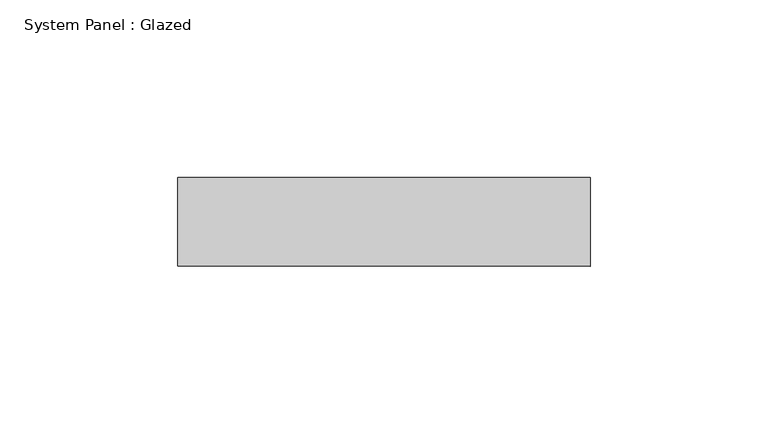
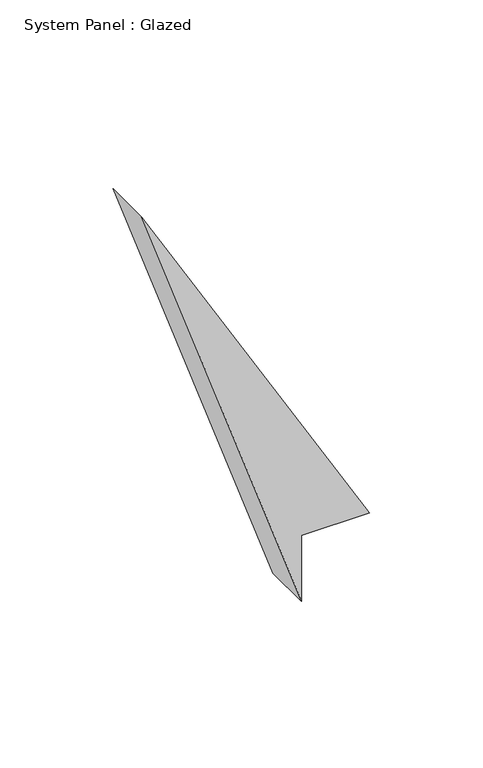
"""IFC4 building model written with IfcOpenShell, lengths in millimetres: plate geometry, System Panel : Glazed."""

from ifc_helpers import new_model, si_unit, frame, origin, place, context, project, spatial, polyline, outline, extrude, source, transform, mapped, element, save


def system_panel_glazed_54b3e94c(model_context):
    return source(origin(), model_context, "Body", "SweptSolid", [
        extrude(outline(polyline([(0.0, 23.3505759), (35.3553391, 23.3505759), (35.3553391, 58.0717743), (235.5388878, -58.0717743), (0.0, 23.3505759)])), frame((0.0, -49.5, 0.0), z_axis=(0.0, 1.0, 0.0), x_axis=(0.0, 0.0, 1.0)), (0.0, 0.0, 1.0), 25.0),
    ])


if __name__ == "__main__":
    model = new_model("IFC4")
    model_context = context("Model", 3, world=origin())
    ifc_project = project(units=[si_unit("LENGTHUNIT", "METRE", prefix="MILLI")], contexts=[model_context])
    site = spatial("IfcSite", under=ifc_project)
    building = spatial("IfcBuilding", under=site)
    placement = place(None, origin())
    system_panel_glazed_shape = system_panel_glazed_54b3e94c(model_context)
    element("IfcPlate", 1, ObjectType="System Panel : Glazed", at=placement, inside=building, context=model_context, shape_type="MappedRepresentation", body=[
        mapped(system_panel_glazed_shape, transform((0.0, 0.0, 0.0), x_axis=(1.0, 0.0, 0.0), y_axis=(0.0, 1.0, 0.0), z_axis=(0.0, 0.0, 1.0))),
    ])
    save(model, "model.ifc")

# Revit data of these elements
# Element 1 (IfcPlate, "System Panel : Glazed")
#   Materials on its faces: "Glass"
# Materials
#   "Glass": class "Glass", colour RGB 218 227 224, transparency 0.85, Description = "Soda Lime Glass", Cost = 0
